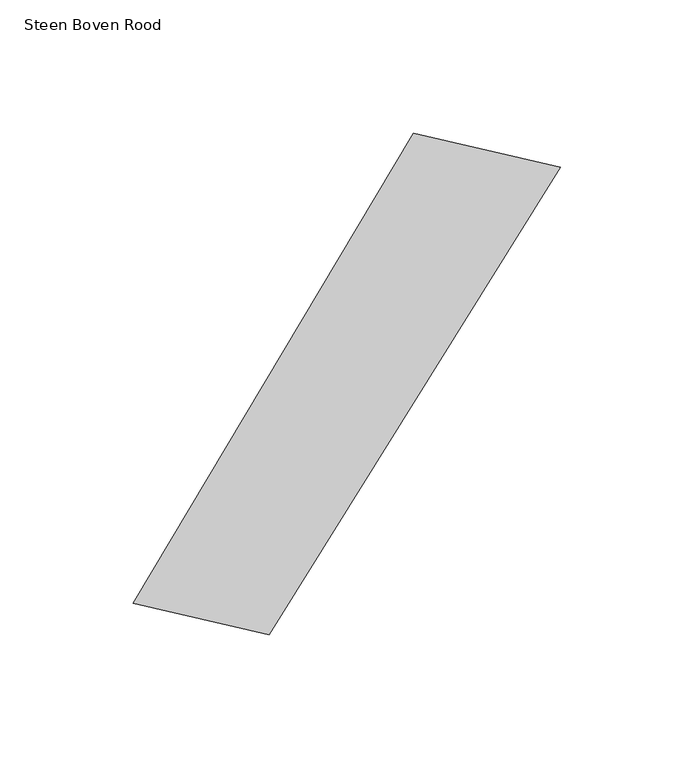
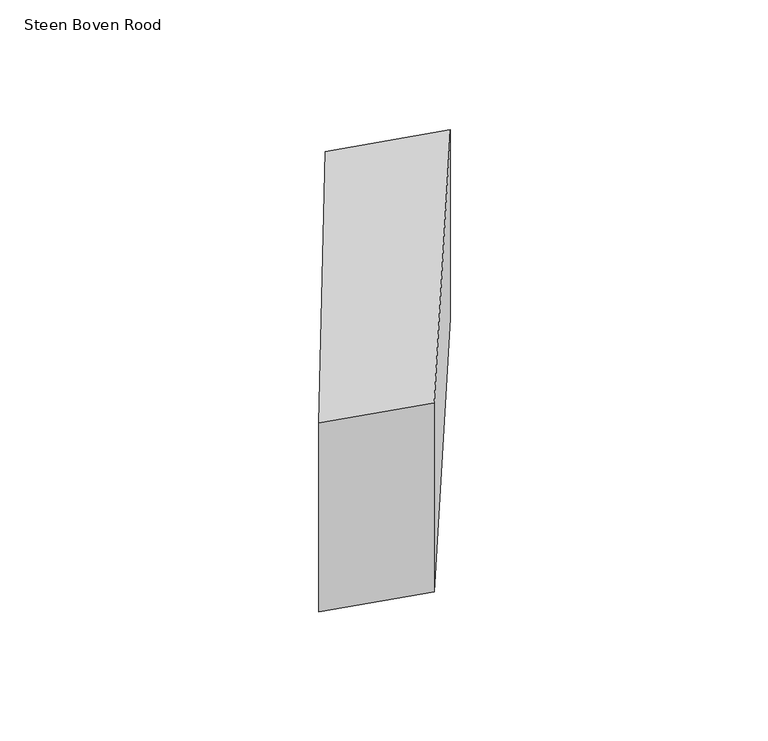
"""IFC4 building model written with IfcOpenShell, lengths in millimetres: proxy geometry, 00_GMA_steen_versie_4 : Steen Boven Rood."""

import ifcopenshell
import ifcopenshell.guid

model = None  # the IFC model being written
_history = None  # IfcOwnerHistory: only IFC2X3 demands one
_inside = {}  # id of a spatial element -> (the spatial element, [elements in it])
_under = {}  # id of a project, library or spatial element -> (it, [spatial elements below it])
_declared = {}  # id of a project -> (the project, [libraries it declares])
_typed = {}  # id of a type object -> (the type object, [elements of that type])
_made_of = {}  # id of a material, layer set ... -> (it, [elements and type objects made of it])


def new_model(schema):
    """Start an empty IFC model of exactly this schema.

    Asked for "IFC4X3", IfcOpenShell would pick the latest addendum, in which some entities
    have other attributes; the version numbers below select the first issue.
    IFC2X3 requires an IfcOwnerHistory on every rooted entity: one is made here for all.
    """
    global model, _history
    if schema == "IFC4X3":
        model = ifcopenshell.file(schema_version=(4, 3, 0, 0))
    else:
        model = ifcopenshell.file(schema=schema)
    _inside.clear()
    _under.clear()
    _declared.clear()
    _typed.clear()
    _made_of.clear()
    _history = None
    if model.schema == "IFC2X3":
        org = make("IfcOrganization", Name="unknown")
        user = make(
            "IfcPersonAndOrganization",
            ThePerson=make("IfcPerson", FamilyName="unknown"),
            TheOrganization=org,
        )
        app = make(
            "IfcApplication",
            ApplicationDeveloper=org,
            Version="unknown",
            ApplicationFullName="unknown",
            ApplicationIdentifier="unknown",
        )
        _history = make(
            "IfcOwnerHistory",
            OwningUser=user,
            OwningApplication=app,
            ChangeAction="ADDED",
            CreationDate=0,
        )
    return model


def make(cls, **values):
    """One entity of the class cls with the attributes given. An attribute that is None is left unset."""
    return model.create_entity(
        cls, **{name: value for name, value in values.items() if value is not None}
    )


def rooted(cls, **values):
    """An entity with a GlobalId (a new one), such as an element, a storey or a relation."""
    return make(cls, GlobalId=ifcopenshell.guid.new(), OwnerHistory=_history, **values)


def si_unit(unit_type, name, prefix=None):
    """IfcSIUnit, for example si_unit("LENGTHUNIT", "METRE", prefix="MILLI")."""
    return make("IfcSIUnit", UnitType=unit_type, Prefix=prefix, Name=name)


def assignment(units):
    """IfcUnitAssignment: the units of a project."""
    return None if units is None else make("IfcUnitAssignment", Units=units)


def point(xyz):
    """IfcCartesianPoint."""
    return None if xyz is None else make("IfcCartesianPoint", Coordinates=xyz)


def direction(xyz):
    """IfcDirection."""
    return None if xyz is None else make("IfcDirection", DirectionRatios=xyz)


def frame(location, z_axis=None, x_axis=None):
    """IfcAxis2Placement3D, a coordinate frame: its origin and axes. An axis left out is left unset."""
    return make(
        "IfcAxis2Placement3D",
        Location=point(location),
        Axis=direction(z_axis),
        RefDirection=direction(x_axis),
    )


def origin():
    """The frame at (0, 0, 0) with its axes left unset."""
    return frame((0.0, 0.0, 0.0))


def origin_with_axes():
    """The frame at (0, 0, 0) with the z axis (0, 0, 1) and the x axis (1, 0, 0) written out."""
    return frame((0.0, 0.0, 0.0), z_axis=(0.0, 0.0, 1.0), x_axis=(1.0, 0.0, 0.0))


def place(relative_to, where):
    """IfcLocalPlacement: puts the frame where relative to a parent placement (None: the world)."""
    return make(
        "IfcLocalPlacement", PlacementRelTo=relative_to, RelativePlacement=where
    )


def context(
    kind, dimensions, precision=None, world=None, true_north=None, identifier=None
):
    """IfcGeometricRepresentationContext, for example the 3D "Model" context."""
    return make(
        "IfcGeometricRepresentationContext",
        ContextIdentifier=identifier,
        ContextType=kind,
        CoordinateSpaceDimension=dimensions,
        Precision=precision,
        WorldCoordinateSystem=world,
        TrueNorth=true_north,
    )


def project(units=None, contexts=None):
    """IfcProject with its units and contexts."""
    return rooted(
        "IfcProject",
        Name="project",
        RepresentationContexts=contexts,
        UnitsInContext=assignment(units),
    )


def spatial(cls, under=None, at=None, **own):
    """A site, building, storey or space (cls), placed at a placement, below another one or the project."""
    s = rooted(cls, ObjectPlacement=at, **own)
    if under is not None:
        _under.setdefault(under.id(), (under, []))[1].append(s)
    return s


def polyline(points):
    """IfcPolyline through the points."""
    return make("IfcPolyline", Points=[point(p) for p in points])


def outline(outer, holes=None, kind="AREA"):
    """IfcArbitraryClosedProfileDef: a profile drawn as a closed curve; with holes, ...WithVoids."""
    if holes is None:
        return make("IfcArbitraryClosedProfileDef", ProfileType=kind, OuterCurve=outer)
    return make(
        "IfcArbitraryProfileDefWithVoids",
        ProfileType=kind,
        OuterCurve=outer,
        InnerCurves=holes,
    )


def extrude(swept, where, along, depth):
    """IfcExtrudedAreaSolid: the profile swept, set in the frame where, extruded along a direction by depth."""
    return make(
        "IfcExtrudedAreaSolid",
        SweptArea=swept,
        Position=where,
        ExtrudedDirection=direction(along),
        Depth=depth,
    )


def shape(context_of_items, identifier, shape_type, items):
    """IfcShapeRepresentation: the items that make up one representation, for example the "Body"."""
    return make(
        "IfcShapeRepresentation",
        ContextOfItems=context_of_items,
        RepresentationIdentifier=identifier,
        RepresentationType=shape_type,
        Items=items,
    )


def source(mapping_origin, context_of_items, identifier, shape_type, items):
    """IfcRepresentationMap: a shape defined once, which mapped items show again and again."""
    return make(
        "IfcRepresentationMap",
        MappingOrigin=mapping_origin,
        MappedRepresentation=shape(context_of_items, identifier, shape_type, items),
    )


def transform(
    local_origin,
    x_axis=None,
    y_axis=None,
    z_axis=None,
    scale=None,
    scale2=None,
    scale3=None,
    uniform=True,
):
    """IfcCartesianTransformationOperator3D, or its non-uniform kind. x_axis, y_axis, z_axis: its Axis1, 2, 3."""
    if uniform:
        return make(
            "IfcCartesianTransformationOperator3D",
            Axis1=direction(x_axis),
            Axis2=direction(y_axis),
            LocalOrigin=point(local_origin),
            Scale=scale,
            Axis3=direction(z_axis),
        )
    return make(
        "IfcCartesianTransformationOperator3DnonUniform",
        Axis1=direction(x_axis),
        Axis2=direction(y_axis),
        LocalOrigin=point(local_origin),
        Scale=scale,
        Axis3=direction(z_axis),
        Scale2=scale2,
        Scale3=scale3,
    )


def mapped(mapping_source, mapping_target):
    """IfcMappedItem: shows the shape of a source again, moved by a transform."""
    return make(
        "IfcMappedItem", MappingSource=mapping_source, MappingTarget=mapping_target
    )


def made_of(thing, what):
    """Note that an element or type object is made of a material, layer set ...; save() writes the relation."""
    if what is not None:
        _made_of.setdefault(what.id(), (what, []))[1].append(thing)
    return thing


def element(
    cls,
    number,
    at=None,
    inside=None,
    cuts=None,
    type_object=None,
    material=None,
    context=None,
    identifier="Body",
    shape_type=None,
    held_by="IfcProductDefinitionShape",
    body=None,
    shapes=None,
    **own,
):
    """One element of the class cls, such as IfcWall. Its Tag is "e" and its number.

    at: its placement. inside: the storey or other place that contains it. cuts: it is an
    opening in that element (IfcRelVoidsElement). A single representation is given by context,
    identifier, shape_type and body (its items); several are given by shapes. held_by: the class
    of the entity that holds the representations. save() writes the other relations.
    """
    e = rooted(cls, Tag="e%d" % number, ObjectPlacement=at, **own)
    if body is not None:
        shapes = [shape(context, identifier, shape_type, body)]
    if shapes is not None:
        e.Representation = make(held_by, Representations=shapes)
    if inside is not None:
        _inside.setdefault(inside.id(), (inside, []))[1].append(e)
    if cuts is not None:
        rooted(
            "IfcRelVoidsElement", RelatingBuildingElement=cuts, RelatedOpeningElement=e
        )
    if type_object is not None:
        _typed.setdefault(type_object.id(), (type_object, []))[1].append(e)
    return made_of(e, material)


def aggregate(whole, parts):
    """IfcRelAggregates: a whole, such as a stair, and the parts it consists of."""
    return rooted("IfcRelAggregates", RelatingObject=whole, RelatedObjects=parts)


def save(model, path):
    """Write the relations noted so far, then the file.

    IfcRelAggregates (storeys below a building ...), IfcRelContainedInSpatialStructure (elements
    in a storey), IfcRelDefinesByType, IfcRelAssociatesMaterial and IfcRelDeclares: one each for
    every whole, place, type object, material and project.
    """
    for whole, parts in _under.values():
        aggregate(whole, parts)
    for where, things in _inside.values():
        rooted(
            "IfcRelContainedInSpatialStructure",
            RelatedElements=things,
            RelatingStructure=where,
        )
    for kind, things in _typed.values():
        rooted("IfcRelDefinesByType", RelatedObjects=things, RelatingType=kind)
    for what, things in _made_of.values():
        rooted("IfcRelAssociatesMaterial", RelatedObjects=things, RelatingMaterial=what)
    for by, libraries in _declared.values():
        rooted("IfcRelDeclares", RelatingContext=by, RelatedDefinitions=libraries)
    model.write(path)


def steen_boven_rood_8568f795(model_context):
    return source(origin(), model_context, "Body", "SweptSolid", [
        extrude(outline(polyline([(156.6622493, 159.4524114), (47.3455083, -15.7737877), (-3.6345471, -4.021661), (101.4373315, 172.1535752), (156.6622493, 159.4524114)])), origin_with_axes(), (0.0, 0.0, 1.0), 100.0),
    ])


if __name__ == "__main__":
    model = new_model("IFC4")
    model_context = context("Model", 3, world=origin())
    ifc_project = project(units=[si_unit("LENGTHUNIT", "METRE", prefix="MILLI")], contexts=[model_context])
    site = spatial("IfcSite", under=ifc_project)
    building = spatial("IfcBuilding", under=site)
    placement = place(None, origin())
    steen_boven_rood_shape = steen_boven_rood_8568f795(model_context)
    element("IfcBuildingElementProxy", 1, Name="00_GMA_steen_versie_4 : Steen Boven Rood", ObjectType="00_GMA_steen_versie_4 : Steen Boven Rood", at=placement, inside=building, context=model_context, shape_type="MappedRepresentation", body=[
        mapped(steen_boven_rood_shape, transform((0.0, 0.0, 0.0), x_axis=(1.0, 0.0, 0.0), y_axis=(0.0, 1.0, 0.0), z_axis=(0.0, 0.0, 1.0))),
    ])
    save(model, "model.ifc")

# Revit data of these elements
# Type "00_GMA_steen_versie_4 : Steen Boven Rood"
#   StootVoegHalfBoven [instance default] = 5 mm
#   StootVoegHalf [instance default] = 5 mm
#   StootVoegBreedteOnder = 10 mm
#   StootVoegBreedteBoven = 10 mm
#   Steendikte = 100 mm
#   LintVoegOnderHalf = 5 mm
#   LintVoegOnder = 10 mm
#   LintVoegBovenHalf = 0 mm
#   LintVoegBoven = 0 mm
#   materiaal = 21_steen_rood
#   MateriaalVoeg = none
#   Default Elevation = 0
# Element 1 (IfcBuildingElementProxy, "00_GMA_steen_versie_4 : Steen Boven Rood")
#   Materials on its faces: "21_steen_rood"
# Materials
#   "21_steen_rood": class "Unassigned", colour RGB 213 111 43, transparency 0, Cost = 0
